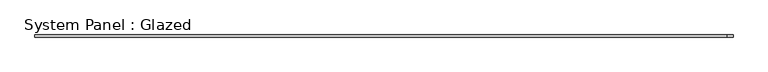
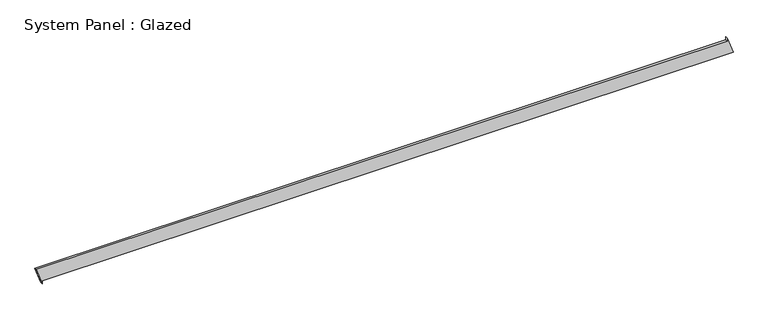
"""IFC4 building model written with IfcOpenShell, lengths in millimetres: plate geometry, System Panel : Glazed."""

from ifc_helpers import new_model, si_unit, frame, origin, place, context, project, spatial, polyline, outline, extrude, source, transform, mapped, element, save


def system_panel_glazed_e03a77ac(model_context):
    return source(origin(), model_context, "Body", "SweptSolid", [
        extrude(outline(polyline([(0.0, -3958.6046047), (35.3553391, -3958.6046047), (35.3553391, 4028.4340057), (234.3037327, 3958.6865343), (198.9483937, 3958.6866872), (198.9138478, -4028.4340057), (0.0, -3958.6046047)])), frame((0.0, -49.5, 0.0), z_axis=(0.0, 1.0, 0.0), x_axis=(0.0, 0.0, 1.0)), (0.0, 0.0, 1.0), 25.0),
    ])


if __name__ == "__main__":
    model = new_model("IFC4")
    model_context = context("Model", 3, world=origin())
    ifc_project = project(units=[si_unit("LENGTHUNIT", "METRE", prefix="MILLI")], contexts=[model_context])
    site = spatial("IfcSite", under=ifc_project)
    building = spatial("IfcBuilding", under=site)
    placement = place(None, origin())
    system_panel_glazed_shape = system_panel_glazed_e03a77ac(model_context)
    element("IfcPlate", 1, ObjectType="System Panel : Glazed", at=placement, inside=building, context=model_context, shape_type="MappedRepresentation", body=[
        mapped(system_panel_glazed_shape, transform((0.0, 0.0, 0.0), x_axis=(1.0, 0.0, 0.0), y_axis=(0.0, 1.0, 0.0), z_axis=(0.0, 0.0, 1.0))),
    ])
    save(model, "model.ifc")

# Revit data of these elements
# Element 1 (IfcPlate, "System Panel : Glazed")
#   Materials on its faces: "Glass"
# Materials
#   "Glass": class "Glass", colour RGB 218 227 224, transparency 0.85, Description = "Soda Lime Glass", Cost = 0
